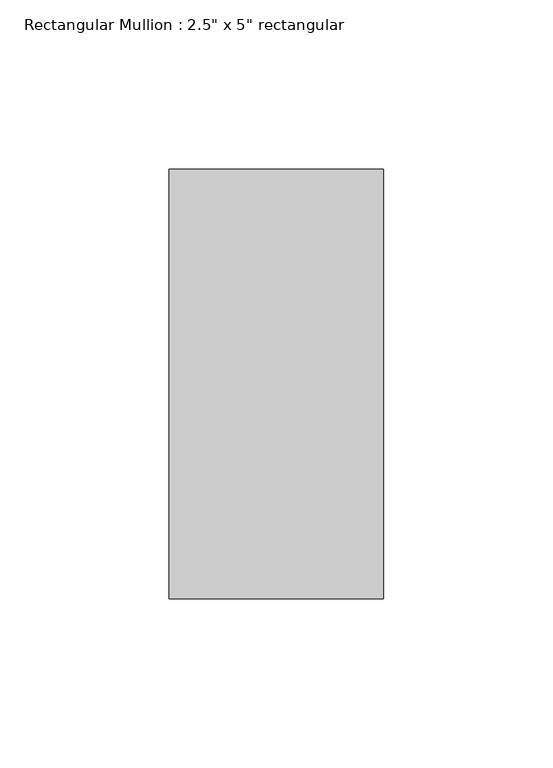
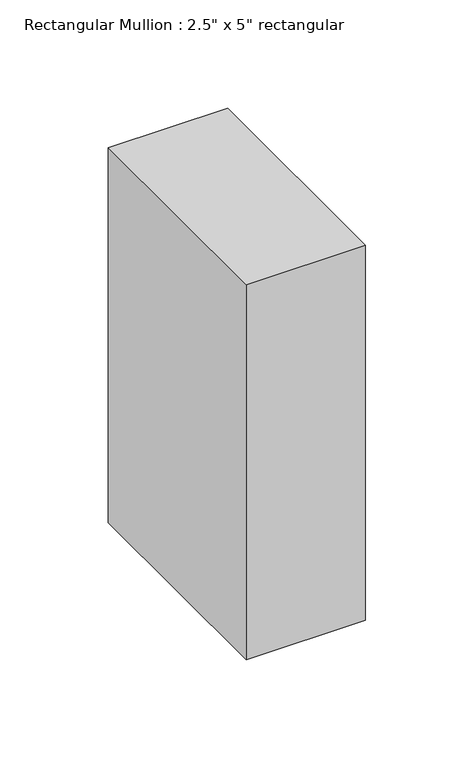
"""IFC4 building model written with IfcOpenShell, lengths in millimetres: member geometry."""

import ifcopenshell
import ifcopenshell.guid

model = None  # the IFC model being written
_history = None  # IfcOwnerHistory: only IFC2X3 demands one
_inside = {}  # id of a spatial element -> (the spatial element, [elements in it])
_under = {}  # id of a project, library or spatial element -> (it, [spatial elements below it])
_declared = {}  # id of a project -> (the project, [libraries it declares])
_typed = {}  # id of a type object -> (the type object, [elements of that type])
_made_of = {}  # id of a material, layer set ... -> (it, [elements and type objects made of it])


def new_model(schema):
    """Start an empty IFC model of exactly this schema.

    Asked for "IFC4X3", IfcOpenShell would pick the latest addendum, in which some entities
    have other attributes; the version numbers below select the first issue.
    IFC2X3 requires an IfcOwnerHistory on every rooted entity: one is made here for all.
    """
    global model, _history
    if schema == "IFC4X3":
        model = ifcopenshell.file(schema_version=(4, 3, 0, 0))
    else:
        model = ifcopenshell.file(schema=schema)
    _inside.clear()
    _under.clear()
    _declared.clear()
    _typed.clear()
    _made_of.clear()
    _history = None
    if model.schema == "IFC2X3":
        org = make("IfcOrganization", Name="unknown")
        user = make(
            "IfcPersonAndOrganization",
            ThePerson=make("IfcPerson", FamilyName="unknown"),
            TheOrganization=org,
        )
        app = make(
            "IfcApplication",
            ApplicationDeveloper=org,
            Version="unknown",
            ApplicationFullName="unknown",
            ApplicationIdentifier="unknown",
        )
        _history = make(
            "IfcOwnerHistory",
            OwningUser=user,
            OwningApplication=app,
            ChangeAction="ADDED",
            CreationDate=0,
        )
    return model


def make(cls, **values):
    """One entity of the class cls with the attributes given. An attribute that is None is left unset."""
    return model.create_entity(
        cls, **{name: value for name, value in values.items() if value is not None}
    )


def rooted(cls, **values):
    """An entity with a GlobalId (a new one), such as an element, a storey or a relation."""
    return make(cls, GlobalId=ifcopenshell.guid.new(), OwnerHistory=_history, **values)


def si_unit(unit_type, name, prefix=None):
    """IfcSIUnit, for example si_unit("LENGTHUNIT", "METRE", prefix="MILLI")."""
    return make("IfcSIUnit", UnitType=unit_type, Prefix=prefix, Name=name)


def assignment(units):
    """IfcUnitAssignment: the units of a project."""
    return None if units is None else make("IfcUnitAssignment", Units=units)


def point(xyz):
    """IfcCartesianPoint."""
    return None if xyz is None else make("IfcCartesianPoint", Coordinates=xyz)


def direction(xyz):
    """IfcDirection."""
    return None if xyz is None else make("IfcDirection", DirectionRatios=xyz)


def frame(location, z_axis=None, x_axis=None):
    """IfcAxis2Placement3D, a coordinate frame: its origin and axes. An axis left out is left unset."""
    return make(
        "IfcAxis2Placement3D",
        Location=point(location),
        Axis=direction(z_axis),
        RefDirection=direction(x_axis),
    )


def origin():
    """The frame at (0, 0, 0) with its axes left unset."""
    return frame((0.0, 0.0, 0.0))


def place(relative_to, where):
    """IfcLocalPlacement: puts the frame where relative to a parent placement (None: the world)."""
    return make(
        "IfcLocalPlacement", PlacementRelTo=relative_to, RelativePlacement=where
    )


def context(
    kind, dimensions, precision=None, world=None, true_north=None, identifier=None
):
    """IfcGeometricRepresentationContext, for example the 3D "Model" context."""
    return make(
        "IfcGeometricRepresentationContext",
        ContextIdentifier=identifier,
        ContextType=kind,
        CoordinateSpaceDimension=dimensions,
        Precision=precision,
        WorldCoordinateSystem=world,
        TrueNorth=true_north,
    )


def project(units=None, contexts=None):
    """IfcProject with its units and contexts."""
    return rooted(
        "IfcProject",
        Name="project",
        RepresentationContexts=contexts,
        UnitsInContext=assignment(units),
    )


def spatial(cls, under=None, at=None, **own):
    """A site, building, storey or space (cls), placed at a placement, below another one or the project."""
    s = rooted(cls, ObjectPlacement=at, **own)
    if under is not None:
        _under.setdefault(under.id(), (under, []))[1].append(s)
    return s


def polyline(points):
    """IfcPolyline through the points."""
    return make("IfcPolyline", Points=[point(p) for p in points])


def outline(outer, holes=None, kind="AREA"):
    """IfcArbitraryClosedProfileDef: a profile drawn as a closed curve; with holes, ...WithVoids."""
    if holes is None:
        return make("IfcArbitraryClosedProfileDef", ProfileType=kind, OuterCurve=outer)
    return make(
        "IfcArbitraryProfileDefWithVoids",
        ProfileType=kind,
        OuterCurve=outer,
        InnerCurves=holes,
    )


def extrude(swept, where, along, depth):
    """IfcExtrudedAreaSolid: the profile swept, set in the frame where, extruded along a direction by depth."""
    return make(
        "IfcExtrudedAreaSolid",
        SweptArea=swept,
        Position=where,
        ExtrudedDirection=direction(along),
        Depth=depth,
    )


def shape(context_of_items, identifier, shape_type, items):
    """IfcShapeRepresentation: the items that make up one representation, for example the "Body"."""
    return make(
        "IfcShapeRepresentation",
        ContextOfItems=context_of_items,
        RepresentationIdentifier=identifier,
        RepresentationType=shape_type,
        Items=items,
    )


def source(mapping_origin, context_of_items, identifier, shape_type, items):
    """IfcRepresentationMap: a shape defined once, which mapped items show again and again."""
    return make(
        "IfcRepresentationMap",
        MappingOrigin=mapping_origin,
        MappedRepresentation=shape(context_of_items, identifier, shape_type, items),
    )


def transform(
    local_origin,
    x_axis=None,
    y_axis=None,
    z_axis=None,
    scale=None,
    scale2=None,
    scale3=None,
    uniform=True,
):
    """IfcCartesianTransformationOperator3D, or its non-uniform kind. x_axis, y_axis, z_axis: its Axis1, 2, 3."""
    if uniform:
        return make(
            "IfcCartesianTransformationOperator3D",
            Axis1=direction(x_axis),
            Axis2=direction(y_axis),
            LocalOrigin=point(local_origin),
            Scale=scale,
            Axis3=direction(z_axis),
        )
    return make(
        "IfcCartesianTransformationOperator3DnonUniform",
        Axis1=direction(x_axis),
        Axis2=direction(y_axis),
        LocalOrigin=point(local_origin),
        Scale=scale,
        Axis3=direction(z_axis),
        Scale2=scale2,
        Scale3=scale3,
    )


def mapped(mapping_source, mapping_target):
    """IfcMappedItem: shows the shape of a source again, moved by a transform."""
    return make(
        "IfcMappedItem", MappingSource=mapping_source, MappingTarget=mapping_target
    )


def made_of(thing, what):
    """Note that an element or type object is made of a material, layer set ...; save() writes the relation."""
    if what is not None:
        _made_of.setdefault(what.id(), (what, []))[1].append(thing)
    return thing


def element(
    cls,
    number,
    at=None,
    inside=None,
    cuts=None,
    type_object=None,
    material=None,
    context=None,
    identifier="Body",
    shape_type=None,
    held_by="IfcProductDefinitionShape",
    body=None,
    shapes=None,
    **own,
):
    """One element of the class cls, such as IfcWall. Its Tag is "e" and its number.

    at: its placement. inside: the storey or other place that contains it. cuts: it is an
    opening in that element (IfcRelVoidsElement). A single representation is given by context,
    identifier, shape_type and body (its items); several are given by shapes. held_by: the class
    of the entity that holds the representations. save() writes the other relations.
    """
    e = rooted(cls, Tag="e%d" % number, ObjectPlacement=at, **own)
    if body is not None:
        shapes = [shape(context, identifier, shape_type, body)]
    if shapes is not None:
        e.Representation = make(held_by, Representations=shapes)
    if inside is not None:
        _inside.setdefault(inside.id(), (inside, []))[1].append(e)
    if cuts is not None:
        rooted(
            "IfcRelVoidsElement", RelatingBuildingElement=cuts, RelatedOpeningElement=e
        )
    if type_object is not None:
        _typed.setdefault(type_object.id(), (type_object, []))[1].append(e)
    return made_of(e, material)


def aggregate(whole, parts):
    """IfcRelAggregates: a whole, such as a stair, and the parts it consists of."""
    return rooted("IfcRelAggregates", RelatingObject=whole, RelatedObjects=parts)


def save(model, path):
    """Write the relations noted so far, then the file.

    IfcRelAggregates (storeys below a building ...), IfcRelContainedInSpatialStructure (elements
    in a storey), IfcRelDefinesByType, IfcRelAssociatesMaterial and IfcRelDeclares: one each for
    every whole, place, type object, material and project.
    """
    for whole, parts in _under.values():
        aggregate(whole, parts)
    for where, things in _inside.values():
        rooted(
            "IfcRelContainedInSpatialStructure",
            RelatedElements=things,
            RelatingStructure=where,
        )
    for kind, things in _typed.values():
        rooted("IfcRelDefinesByType", RelatedObjects=things, RelatingType=kind)
    for what, things in _made_of.values():
        rooted("IfcRelAssociatesMaterial", RelatedObjects=things, RelatingMaterial=what)
    for by, libraries in _declared.values():
        rooted("IfcRelDeclares", RelatingContext=by, RelatedDefinitions=libraries)
    model.write(path)


def member_38b8e9cb(model_context):
    return source(origin(), model_context, "Body", "SweptSolid", [
        extrude(outline(polyline([(31.75, 63.5), (31.75, -63.5), (-31.75, -63.5), (-31.75, 63.5), (31.75, 63.5)])), frame((0.0, 0.0, -210.9151287), z_axis=(0.0, 0.0, 1.0), x_axis=(1.0, 0.0, 0.0)), (0.0, 0.0, 1.0), 210.9151287),
    ])


if __name__ == "__main__":
    model = new_model("IFC4")
    model_context = context("Model", 3, world=origin())
    ifc_project = project(units=[si_unit("LENGTHUNIT", "METRE", prefix="MILLI")], contexts=[model_context])
    site = spatial("IfcSite", under=ifc_project)
    building = spatial("IfcBuilding", under=site)
    placement = place(None, origin())
    member_shape = member_38b8e9cb(model_context)
    element("IfcMember", 1, ObjectType="Rectangular Mullion : 2.5\" x 5\" rectangular", at=placement, inside=building, context=model_context, shape_type="MappedRepresentation", body=[
        mapped(member_shape, transform((0.0, 0.0, 0.0), x_axis=(1.0, 0.0, 0.0), y_axis=(0.0, 1.0, 0.0), z_axis=(0.0, 0.0, 1.0))),
    ])
    save(model, "model.ifc")

# Revit data of these elements
# Type "Rectangular Mullion : 2.5\" x 5\" rectangular"
#   built-in parameter 1007304 = 0.416667 (stored number, unit not read)
#   built-in parameter 1007301 = 0.104167 (stored number, unit not read)
#   built-in parameter 1007300 = 0.104167 (stored number, unit not read)
# Element 1 (IfcMember, "Rectangular Mullion : 2.5\" x 5\" rectangular")
#   Materials on its faces: "Metal - Aluminum"
# Materials
#   "Metal - Aluminum": class "Metal", colour RGB 140 140 140, transparency 0
